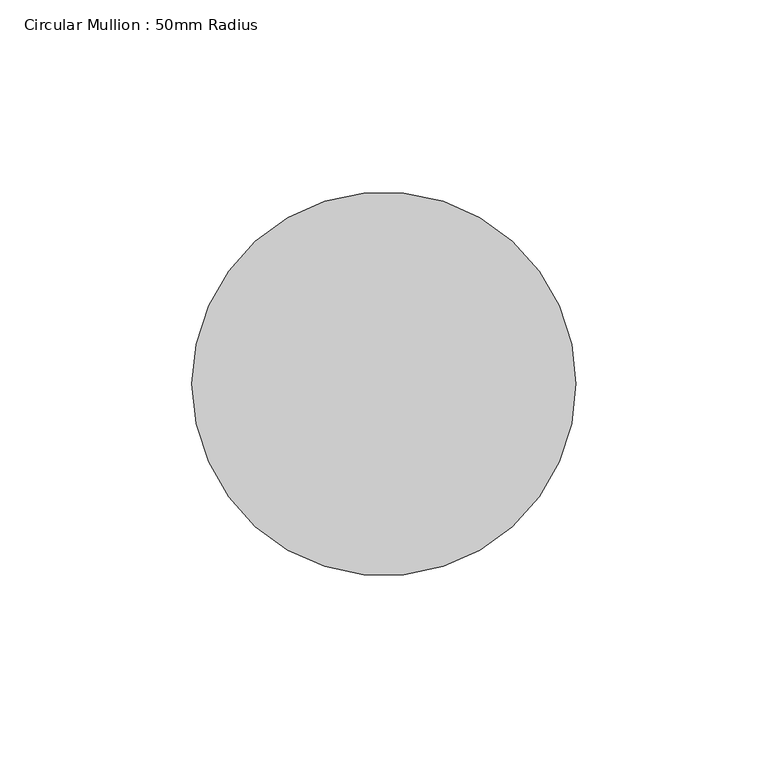
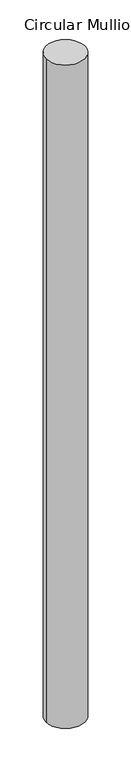
"""IFC4 building model written with IfcOpenShell, lengths in millimetres: member geometry, Circular Mullion : 50mm Radius."""

from ifc_helpers import new_model, si_unit, point, frame, frame_2d, origin, place, context, project, spatial, circle_curve, trimmed, segment, composite_curve, outline, extrude, source, transform, mapped, element, save


def circular_mullion_50mm_radius_efefdd37(model_context):
    return source(origin(), model_context, "Body", "SweptSolid", [
        extrude(outline(composite_curve([segment(trimmed(circle_curve(frame_2d((-50.0, 0.0)), 50.0), [point((0.0, 0.0))], [point((-100.0, 0.0))], False, "CARTESIAN"), True, "CONTINUOUS"), segment(trimmed(circle_curve(frame_2d((-50.0, 0.0)), 50.0), [point((-100.0, 0.0))], [point((0.0, 0.0))], False, "CARTESIAN"), True, "CONTINUOUS")], self_intersect=False)), frame((0.0, 0.0, -1814.6479292), z_axis=(0.0, 0.0, 1.0), x_axis=(1.0, 0.0, 0.0)), (0.0, 0.0, 1.0), 1814.6479292),
    ])


if __name__ == "__main__":
    model = new_model("IFC4")
    model_context = context("Model", 3, world=origin())
    ifc_project = project(units=[si_unit("LENGTHUNIT", "METRE", prefix="MILLI")], contexts=[model_context])
    site = spatial("IfcSite", under=ifc_project)
    building = spatial("IfcBuilding", under=site)
    placement = place(None, origin())
    circular_mullion_50mm_radius_shape = circular_mullion_50mm_radius_efefdd37(model_context)
    element("IfcMember", 1, ObjectType="Circular Mullion : 50mm Radius", at=placement, inside=building, context=model_context, shape_type="MappedRepresentation", body=[
        mapped(circular_mullion_50mm_radius_shape, transform((0.0, 0.0, 0.0), x_axis=(1.0, 0.0, 0.0), y_axis=(0.0, 1.0, 0.0), z_axis=(0.0, 0.0, 1.0))),
    ])
    save(model, "model.ifc")

# Revit data of these elements
# Type "Circular Mullion : 50mm Radius"
#   built-in parameter 1007350 = 0.164042 (stored number, unit not read)
# Element 1 (IfcMember, "Circular Mullion : 50mm Radius")
#   Materials on its faces: "Aluminium"
# Materials
#   "Aluminium": class "Metal", colour RGB 247 247 247, transparency 0, Description = "Aluminium 6061", Cost = 0
